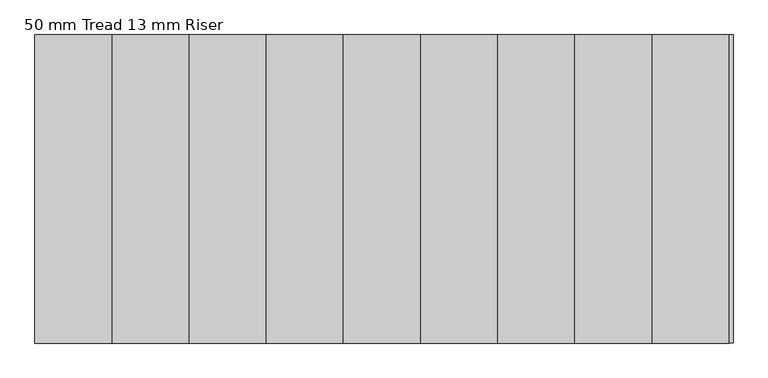
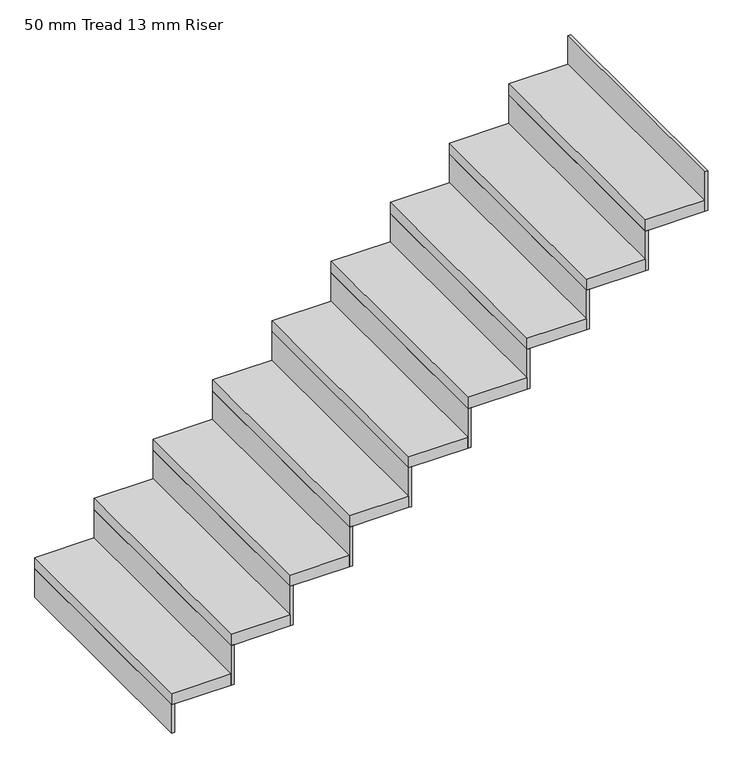
"""IFC4 building model written with IfcOpenShell, lengths in millimetres: stair flight geometry, 50 mm Tread 13 mm Riser."""

from ifc_helpers import new_model, si_unit, frame, origin, origin_with_axes, place, context, project, spatial, polyline, outline, extrude, source, transform, mapped, element, save


def stair_flight_50_mm_tread_13_mm_riser_d0b2eee5(model_context):
    return source(origin(), model_context, "Body", "SweptSolid", [
        extrude(outline(polyline([(7913.2119026, -3663.8378596), (7900.7119026, -3663.8378596), (7900.7119026, -2663.8378596), (7913.2119026, -2663.8378596), (7913.2119026, -3663.8378596)])), origin_with_axes(), (0.0, 0.0, 1.0), 126.4705882),
        extrude(outline(polyline([(8150.7119026, -2663.8378596), (8150.7119026, -3663.8378596), (7900.7119026, -3663.8378596), (7900.7119026, -2663.8378596), (8150.7119026, -2663.8378596)])), frame((0.0, 0.0, 126.4705882), z_axis=(0.0, 0.0, 1.0), x_axis=(1.0, 0.0, 0.0)), (0.0, 0.0, 1.0), 50.0),
        extrude(outline(polyline([(8163.2119026, -3663.8378596), (8150.7119026, -3663.8378596), (8150.7119026, -2663.8378596), (8163.2119026, -2663.8378596), (8163.2119026, -3663.8378596)])), frame((0.0, 0.0, 126.4705882), z_axis=(0.0, 0.0, 1.0), x_axis=(1.0, 0.0, 0.0)), (0.0, 0.0, 1.0), 176.4705882),
        extrude(outline(polyline([(8400.7119026, -2663.8378596), (8400.7119026, -3663.8378596), (8150.7119026, -3663.8378596), (8150.7119026, -2663.8378596), (8400.7119026, -2663.8378596)])), frame((0.0, 0.0, 302.9411765), z_axis=(0.0, 0.0, 1.0), x_axis=(1.0, 0.0, 0.0)), (0.0, 0.0, 1.0), 50.0),
        extrude(outline(polyline([(8413.2119026, -3663.8378596), (8400.7119026, -3663.8378596), (8400.7119026, -2663.8378596), (8413.2119026, -2663.8378596), (8413.2119026, -3663.8378596)])), frame((0.0, 0.0, 302.9411765), z_axis=(0.0, 0.0, 1.0), x_axis=(1.0, 0.0, 0.0)), (0.0, 0.0, 1.0), 176.4705882),
        extrude(outline(polyline([(8650.7119026, -2663.8378596), (8650.7119026, -3663.8378596), (8400.7119026, -3663.8378596), (8400.7119026, -2663.8378596), (8650.7119026, -2663.8378596)])), frame((0.0, 0.0, 479.4117647), z_axis=(0.0, 0.0, 1.0), x_axis=(1.0, 0.0, 0.0)), (0.0, 0.0, 1.0), 50.0),
        extrude(outline(polyline([(8663.2119026, -3663.8378596), (8650.7119026, -3663.8378596), (8650.7119026, -2663.8378596), (8663.2119026, -2663.8378596), (8663.2119026, -3663.8378596)])), frame((0.0, 0.0, 479.4117647), z_axis=(0.0, 0.0, 1.0), x_axis=(1.0, 0.0, 0.0)), (0.0, 0.0, 1.0), 176.4705882),
        extrude(outline(polyline([(8900.7119026, -2663.8378596), (8900.7119026, -3663.8378596), (8650.7119026, -3663.8378596), (8650.7119026, -2663.8378596), (8900.7119026, -2663.8378596)])), frame((0.0, 0.0, 655.8823529), z_axis=(0.0, 0.0, 1.0), x_axis=(1.0, 0.0, 0.0)), (0.0, 0.0, 1.0), 50.0),
        extrude(outline(polyline([(8913.2119026, -3663.8378596), (8900.7119026, -3663.8378596), (8900.7119026, -2663.8378596), (8913.2119026, -2663.8378596), (8913.2119026, -3663.8378596)])), frame((0.0, 0.0, 655.8823529), z_axis=(0.0, 0.0, 1.0), x_axis=(1.0, 0.0, 0.0)), (0.0, 0.0, 1.0), 176.4705882),
        extrude(outline(polyline([(9150.7119026, -2663.8378596), (9150.7119026, -3663.8378596), (8900.7119026, -3663.8378596), (8900.7119026, -2663.8378596), (9150.7119026, -2663.8378596)])), frame((0.0, 0.0, 832.3529412), z_axis=(0.0, 0.0, 1.0), x_axis=(1.0, 0.0, 0.0)), (0.0, 0.0, 1.0), 50.0),
        extrude(outline(polyline([(9163.2119026, -3663.8378596), (9150.7119026, -3663.8378596), (9150.7119026, -2663.8378596), (9163.2119026, -2663.8378596), (9163.2119026, -3663.8378596)])), frame((0.0, 0.0, 832.3529412), z_axis=(0.0, 0.0, 1.0), x_axis=(1.0, 0.0, 0.0)), (0.0, 0.0, 1.0), 176.4705882),
        extrude(outline(polyline([(9400.7119026, -2663.8378596), (9400.7119026, -3663.8378596), (9150.7119026, -3663.8378596), (9150.7119026, -2663.8378596), (9400.7119026, -2663.8378596)])), frame((0.0, 0.0, 1008.8235294), z_axis=(0.0, 0.0, 1.0), x_axis=(1.0, 0.0, 0.0)), (0.0, 0.0, 1.0), 50.0),
        extrude(outline(polyline([(9413.2119026, -3663.8378596), (9400.7119026, -3663.8378596), (9400.7119026, -2663.8378596), (9413.2119026, -2663.8378596), (9413.2119026, -3663.8378596)])), frame((0.0, 0.0, 1008.8235294), z_axis=(0.0, 0.0, 1.0), x_axis=(1.0, 0.0, 0.0)), (0.0, 0.0, 1.0), 176.4705882),
        extrude(outline(polyline([(9650.7119026, -2663.8378596), (9650.7119026, -3663.8378596), (9400.7119026, -3663.8378596), (9400.7119026, -2663.8378596), (9650.7119026, -2663.8378596)])), frame((0.0, 0.0, 1185.2941176), z_axis=(0.0, 0.0, 1.0), x_axis=(1.0, 0.0, 0.0)), (0.0, 0.0, 1.0), 50.0),
        extrude(outline(polyline([(9663.2119026, -3663.8378596), (9650.7119026, -3663.8378596), (9650.7119026, -2663.8378596), (9663.2119026, -2663.8378596), (9663.2119026, -3663.8378596)])), frame((0.0, 0.0, 1185.2941176), z_axis=(0.0, 0.0, 1.0), x_axis=(1.0, 0.0, 0.0)), (0.0, 0.0, 1.0), 176.4705882),
        extrude(outline(polyline([(9900.7119026, -2663.8378596), (9900.7119026, -3663.8378596), (9650.7119026, -3663.8378596), (9650.7119026, -2663.8378596), (9900.7119026, -2663.8378596)])), frame((0.0, 0.0, 1361.7647059), z_axis=(0.0, 0.0, 1.0), x_axis=(1.0, 0.0, 0.0)), (0.0, 0.0, 1.0), 50.0),
        extrude(outline(polyline([(9913.2119026, -3663.8378596), (9900.7119026, -3663.8378596), (9900.7119026, -2663.8378596), (9913.2119026, -2663.8378596), (9913.2119026, -3663.8378596)])), frame((0.0, 0.0, 1361.7647059), z_axis=(0.0, 0.0, 1.0), x_axis=(1.0, 0.0, 0.0)), (0.0, 0.0, 1.0), 176.4705882),
        extrude(outline(polyline([(10163.2119026, -3663.8378596), (10150.7119026, -3663.8378596), (10150.7119026, -2663.8378596), (10163.2119026, -2663.8378596), (10163.2119026, -3663.8378596)])), frame((0.0, 0.0, 1538.2352941), z_axis=(0.0, 0.0, 1.0), x_axis=(1.0, 0.0, 0.0)), (0.0, 0.0, 1.0), 176.4705882),
        extrude(outline(polyline([(10150.7119026, -2663.8378596), (10150.7119026, -3663.8378596), (9900.7119026, -3663.8378596), (9900.7119026, -2663.8378596), (10150.7119026, -2663.8378596)])), frame((0.0, 0.0, 1538.2352941), z_axis=(0.0, 0.0, 1.0), x_axis=(1.0, 0.0, 0.0)), (0.0, 0.0, 1.0), 50.0),
    ])


if __name__ == "__main__":
    model = new_model("IFC4")
    model_context = context("Model", 3, world=origin())
    ifc_project = project(units=[si_unit("LENGTHUNIT", "METRE", prefix="MILLI")], contexts=[model_context])
    site = spatial("IfcSite", under=ifc_project)
    building = spatial("IfcBuilding", under=site)
    placement = place(None, origin())
    stair_flight_50_mm_tread_13_mm_riser_shape = stair_flight_50_mm_tread_13_mm_riser_d0b2eee5(model_context)
    element("IfcStairFlight", 1, ObjectType="50 mm Tread 13 mm Riser", at=placement, inside=building, context=model_context, shape_type="MappedRepresentation", body=[
        mapped(stair_flight_50_mm_tread_13_mm_riser_shape, transform((0.0, 0.0, 0.0), x_axis=(1.0, 0.0, 0.0), y_axis=(0.0, 1.0, 0.0), z_axis=(0.0, 0.0, 1.0))),
    ])
    save(model, "model.ifc")
